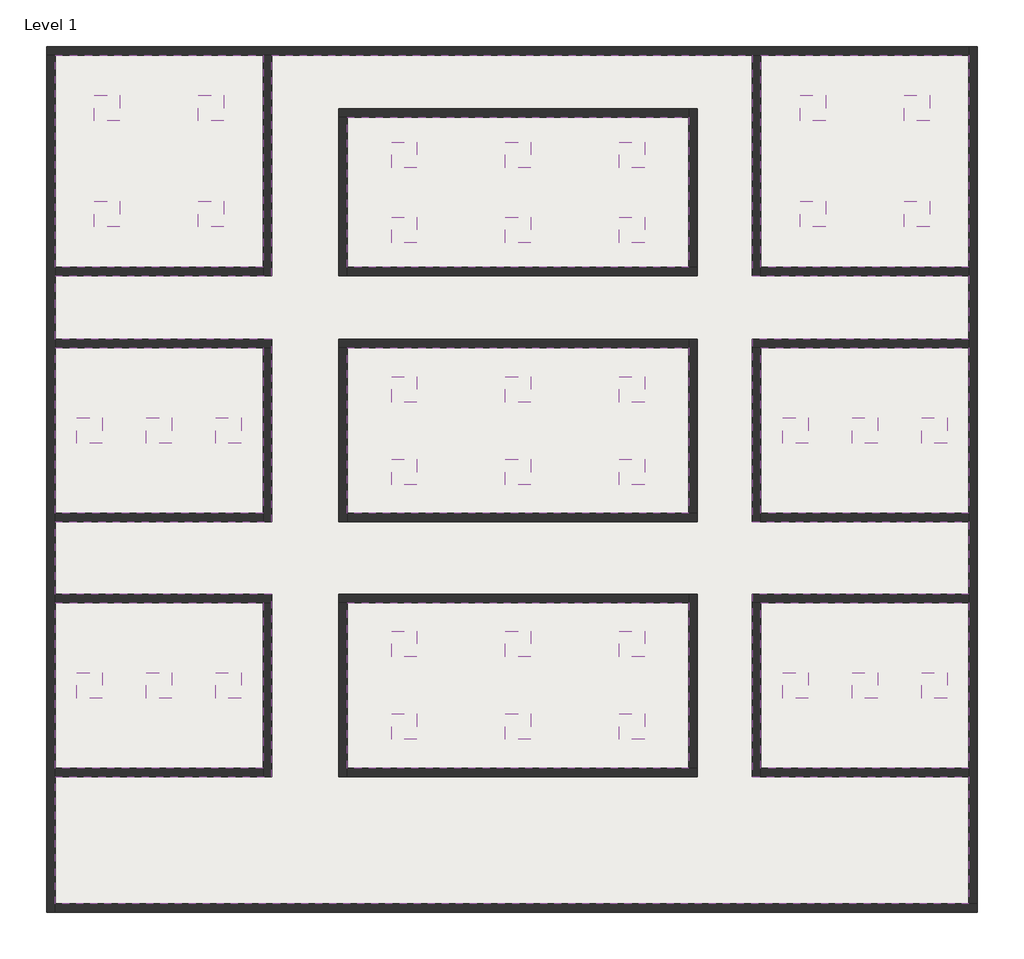
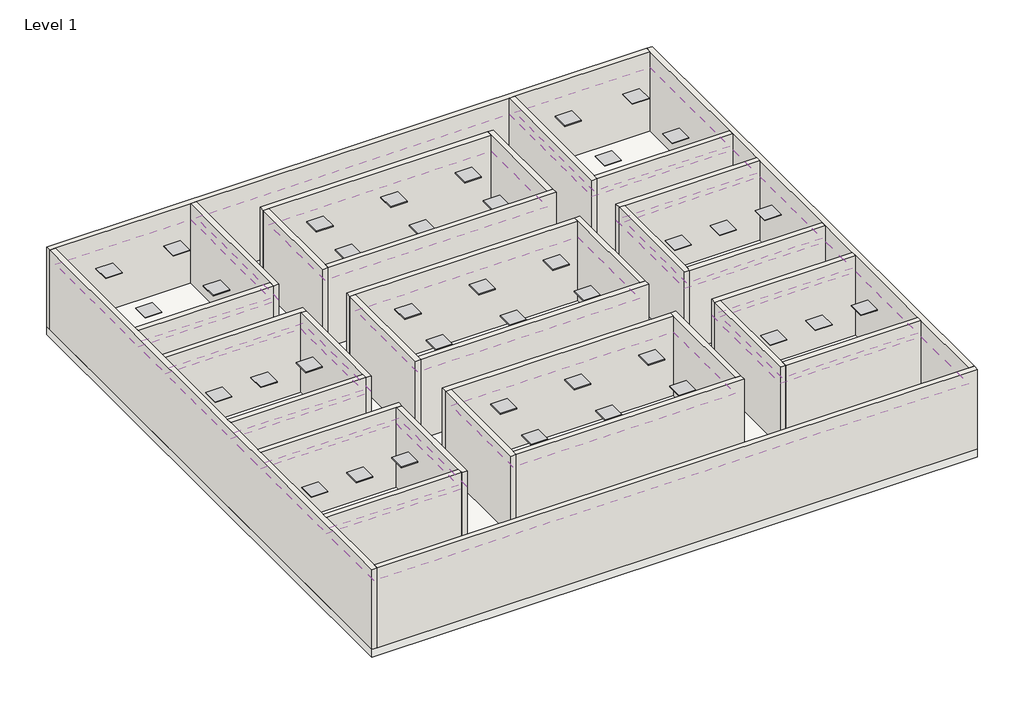
# One storey: 38 light fixtures, 32 walls, 11 coverings, 1 slab.
# Revit data of these elements (continued)
# Element 49 (IfcLightFixture, "Simple Lights : A")
#   Mark = "362"
#   Phase Created = New Construction
# Element 50 (IfcSlab, "Generic - 12\"")
#   Height Offset From Level = 0 m
#   Phase Created = New Construction
#   Materials on its faces: "Default Floor"
# Elements 51, 52, 53, 54, 55, 56, 57, 58, 59, 60, 61, 62, 63, 64, 65, 66, 67, 68, 69, 70, 71, 72, 73, 74, 75, 76, 77, 78, 79, 80, 81, 82 (IfcWall, "Generic - 200mm")
#   Top Offset = 0 m
#   Base Offset = 0 m
#   Unconnected Height = 3 m
#   wall height = 3 m
#   Phase Created = New Construction
#   Base Constraint = Level 1
#   Materials on its faces: "Default Wall"
# Materials
#   "Default": class "Miscellaneous", colour RGB 127 127 127, transparency 0, Cost = 0
#   "Acoustic Ceiling Tile 24 x 48": class "Generic", colour RGB 229 229 229, transparency 0, Description = "Acoustic Ceiling Tile 24 x 48", Cost = 0
#   "Default Floor": class "Miscellaneous", colour RGB 128 128 128, transparency 0, Cost = 0
#   "Default Wall": class "Miscellaneous", colour RGB 128 128 128, transparency 0, Cost = 0
